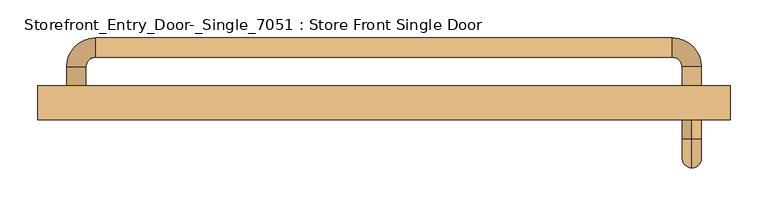
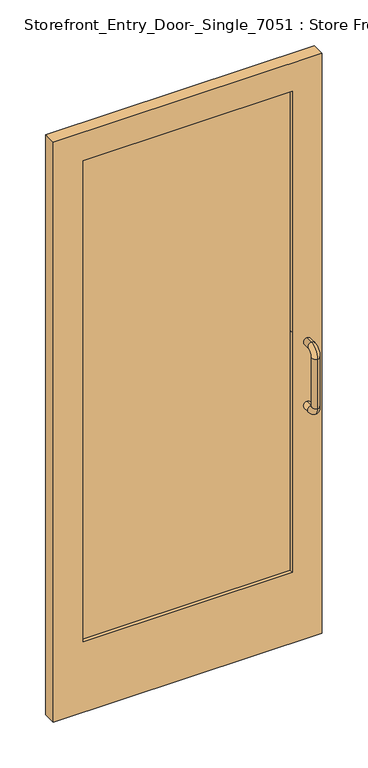
"""IFC4 building model written with IfcOpenShell, lengths in millimetres: door geometry, Storefront_Entry_Door-_Single_7051 : Store Front Single Door."""

from ifc_helpers import new_model, si_unit, point, frame, origin, place, context, project, spatial, polyline, circle_curve, ellipse_curve, trimmed, outline, extrude, source, transform, mapped, element, save
from ifc_brep_helpers import plane_surface, cylinder_surface, revolved_surface, advanced_brep


def storefront_entry_door_single_7051_store_front_single_door_bbd59173(model_context):
    return source(origin(), model_context, "Body", "SolidModel", [
        advanced_brep(
        [(406.4, -50.8, 1054.1), (406.4, -50.8, 1079.5), (406.4, -76.2, 1079.5), (406.4, -76.2, 1054.1), (406.4, -114.3, 1041.4), (406.4, -88.9, 1041.4), (406.4, -114.3, 863.6), (406.4, -88.9, 863.6), (406.4, -76.2, 825.5), (406.4, -76.2, 850.9), (406.4, -50.8, 850.9), (406.4, -50.8, 825.5)],
        [
            (0, 1, circle_curve(frame((406.4, -50.8, 1066.8), z_axis=(0.0, 1.0, 0.0), x_axis=(0.0, 0.0, 1.0)), 12.7)),
            (1, 0, circle_curve(frame((406.4, -50.8, 1066.8), z_axis=(0.0, 1.0, 0.0), x_axis=(0.0, 0.0, 1.0)), 12.7)),
            (1, 2),
            (2, 3, circle_curve(frame((406.4, -76.2, 1066.8), z_axis=(0.0, 1.0, 0.0), x_axis=(0.0, 0.0, 1.0)), 12.7)),
            (3, 0),
            (3, 2, circle_curve(frame((406.4, -76.2, 1066.8), z_axis=(0.0, 1.0, 0.0), x_axis=(0.0, 0.0, 1.0)), 12.7)),
            (4, 5, circle_curve(frame((406.4, -101.6, 1041.4), z_axis=(0.0, 0.0, 1.0), x_axis=(0.0, -1.0, 0.0)), 12.7)),
            (5, 3, circle_curve(frame((406.4, -76.2, 1041.4), z_axis=(-1.0, 0.0, 0.0), x_axis=(0.0, 0.0, 1.0)), 12.7)),
            (2, 4, circle_curve(frame((406.4, -76.2, 1041.4), z_axis=(1.0, 0.0, 0.0), x_axis=(0.0, 0.0, 1.0)), 38.1)),
            (5, 4, circle_curve(frame((406.4, -101.6, 1041.4), z_axis=(0.0, 0.0, 1.0), x_axis=(0.0, -1.0, 0.0)), 12.7)),
            (4, 6),
            (6, 7, circle_curve(frame((406.4, -101.6, 863.6), z_axis=(0.0, 0.0, 1.0), x_axis=(0.0, -1.0, 0.0)), 12.7)),
            (7, 5),
            (7, 6, circle_curve(frame((406.4, -101.6, 863.6), z_axis=(0.0, 0.0, 1.0), x_axis=(0.0, -1.0, 0.0)), 12.7)),
            (8, 9, circle_curve(frame((406.4, -76.2, 838.2), z_axis=(0.0, -1.0, 0.0), x_axis=(0.0, 0.0, -1.0)), 12.7)),
            (9, 7, circle_curve(frame((406.4, -76.2, 863.6), z_axis=(-1.0, 0.0, 0.0), x_axis=(0.0, -1.0, 0.0)), 12.7)),
            (6, 8, circle_curve(frame((406.4, -76.2, 863.6), z_axis=(1.0, 0.0, 0.0), x_axis=(0.0, -1.0, 0.0)), 38.1)),
            (9, 8, circle_curve(frame((406.4, -76.2, 838.2), z_axis=(0.0, -1.0, 0.0), x_axis=(0.0, 0.0, -1.0)), 12.7)),
            (10, 11, circle_curve(frame((406.4, -50.8, 838.2), z_axis=(0.0, 1.0, 0.0), x_axis=(0.0, 0.0, -1.0)), 12.7)),
            (11, 10, circle_curve(frame((406.4, -50.8, 838.2), z_axis=(0.0, 1.0, 0.0), x_axis=(0.0, 0.0, -1.0)), 12.7)),
            (8, 11),
            (10, 9),
        ],
        [
            plane_surface(frame((406.4, -50.8, 1066.8), z_axis=(0.0, 1.0, 0.0), x_axis=(1.0, 0.0, 0.0))),
            cylinder_surface(frame((406.4, -50.8, 1066.8), z_axis=(0.0, 1.0, 0.0), x_axis=(0.0, 0.0, 1.0)), 12.7),
            revolved_surface(trimmed(ellipse_curve(frame((406.4, -76.2, 1066.8), z_axis=(0.0, -1.0, 0.0), x_axis=(0.0, 0.0, 1.0)), 12.7, 12.7), [point((406.4, -76.2, 1054.1))], [point((406.4, -76.2, 1079.5))], True, "CARTESIAN"), (406.4, -76.2, 1041.4), (-1.0, 0.0, 0.0)),
            revolved_surface(trimmed(ellipse_curve(frame((406.4, -76.2, 1066.8), z_axis=(0.0, -1.0, 0.0), x_axis=(0.0, 0.0, 1.0)), 12.7, 12.7), [point((406.4, -76.2, 1079.5))], [point((406.4, -76.2, 1054.1))], True, "CARTESIAN"), (406.4, -76.2, 1041.4), (-1.0, 0.0, 0.0)),
            cylinder_surface(frame((406.4, -101.6, 1041.4), z_axis=(0.0, 0.0, 1.0), x_axis=(0.0, -1.0, 0.0)), 12.7),
            revolved_surface(trimmed(ellipse_curve(frame((406.4, -101.6, 863.6), z_axis=(0.0, 0.0, -1.0), x_axis=(0.0, -1.0, 0.0)), 12.7, 12.7), [point((406.4, -88.9, 863.6))], [point((406.4, -114.3, 863.6))], True, "CARTESIAN"), (406.4, -76.2, 863.6), (-1.0, 0.0, 0.0)),
            revolved_surface(trimmed(ellipse_curve(frame((406.4, -101.6, 863.6), z_axis=(0.0, 0.0, -1.0), x_axis=(0.0, -1.0, 0.0)), 12.7, 12.7), [point((406.4, -114.3, 863.6))], [point((406.4, -88.9, 863.6))], True, "CARTESIAN"), (406.4, -76.2, 863.6), (-1.0, 0.0, 0.0)),
            plane_surface(frame((406.4, -50.8, 838.2), z_axis=(0.0, 1.0, 0.0), x_axis=(1.0, 0.0, 0.0))),
            cylinder_surface(frame((406.4, -76.2, 838.2), z_axis=(0.0, -1.0, 0.0), x_axis=(0.0, 0.0, -1.0)), 12.7),
        ],
        [
            (0, [[1, 2]]),
            (1, [[3, 4, 5, -2]]),
            (1, [[-5, 6, -3, -1]]),
            (2, [[7, 8, -4, 9]]),
            (3, [[10, -9, -6, -8]]),
            (4, [[11, 12, 13, -7]]),
            (4, [[-13, 14, -11, -10]]),
            (5, [[15, 16, -12, 17]]),
            (6, [[18, -17, -14, -16]]),
            (7, [[19, 20]]),
            (8, [[21, -19, 22, -15]]),
            (8, [[-22, -20, -21, -18]]),
        ],
    ),
        advanced_brep(
        [(393.7, -6.35, 1066.8), (419.1, -6.35, 1066.8), (419.1, 19.05, 1066.8), (393.7, 19.05, 1066.8), (381.0, 57.15, 1066.8), (381.0, 31.75, 1066.8), (-381.0, 57.15, 1066.8), (-381.0, 31.75, 1066.8), (-419.1, 19.05, 1066.8), (-393.7, 19.05, 1066.8), (-393.7, -6.35, 1066.8), (-419.1, -6.35, 1066.8)],
        [
            (0, 1, circle_curve(frame((406.4, -6.35, 1066.8), z_axis=(0.0, -1.0, 0.0), x_axis=(1.0, 0.0, 0.0)), 12.7)),
            (1, 0, circle_curve(frame((406.4, -6.35, 1066.8), z_axis=(0.0, -1.0, 0.0), x_axis=(1.0, 0.0, 0.0)), 12.7)),
            (1, 2),
            (2, 3, circle_curve(frame((406.4, 19.05, 1066.8), z_axis=(0.0, -1.0, 0.0), x_axis=(1.0, 0.0, 0.0)), 12.7)),
            (3, 0),
            (3, 2, circle_curve(frame((406.4, 19.05, 1066.8), z_axis=(0.0, -1.0, 0.0), x_axis=(1.0, 0.0, 0.0)), 12.7)),
            (4, 5, circle_curve(frame((381.0, 44.45, 1066.8), z_axis=(1.0, 0.0, 0.0), x_axis=(0.0, 1.0, 0.0)), 12.7)),
            (5, 3, circle_curve(frame((381.0, 19.05, 1066.8), z_axis=(0.0, 0.0, -1.0), x_axis=(1.0, 0.0, 0.0)), 12.7)),
            (2, 4, circle_curve(frame((381.0, 19.05, 1066.8), z_axis=(0.0, 0.0, 1.0), x_axis=(1.0, 0.0, 0.0)), 38.1)),
            (5, 4, circle_curve(frame((381.0, 44.45, 1066.8), z_axis=(1.0, 0.0, 0.0), x_axis=(0.0, 1.0, 0.0)), 12.7)),
            (4, 6),
            (6, 7, circle_curve(frame((-381.0, 44.45, 1066.8), z_axis=(1.0, 0.0, 0.0), x_axis=(0.0, 1.0, 0.0)), 12.7)),
            (7, 5),
            (7, 6, circle_curve(frame((-381.0, 44.45, 1066.8), z_axis=(1.0, 0.0, 0.0), x_axis=(0.0, 1.0, 0.0)), 12.7)),
            (8, 9, circle_curve(frame((-406.4, 19.05, 1066.8), z_axis=(0.0, 1.0, 0.0), x_axis=(-1.0, 0.0, 0.0)), 12.7)),
            (9, 7, circle_curve(frame((-381.0, 19.05, 1066.8), z_axis=(0.0, 0.0, -1.0), x_axis=(0.0, 1.0, 0.0)), 12.7)),
            (6, 8, circle_curve(frame((-381.0, 19.05, 1066.8), z_axis=(0.0, 0.0, 1.0), x_axis=(0.0, 1.0, 0.0)), 38.1)),
            (9, 8, circle_curve(frame((-406.4, 19.05, 1066.8), z_axis=(0.0, 1.0, 0.0), x_axis=(-1.0, 0.0, 0.0)), 12.7)),
            (10, 11, circle_curve(frame((-406.4, -6.35, 1066.8), z_axis=(0.0, -1.0, 0.0), x_axis=(-1.0, 0.0, 0.0)), 12.7)),
            (11, 10, circle_curve(frame((-406.4, -6.35, 1066.8), z_axis=(0.0, -1.0, 0.0), x_axis=(-1.0, 0.0, 0.0)), 12.7)),
            (8, 11),
            (10, 9),
        ],
        [
            plane_surface(frame((406.4, -6.35, 1066.8), z_axis=(0.0, -1.0, 0.0), x_axis=(0.0, 0.0, 1.0))),
            cylinder_surface(frame((406.4, -6.35, 1066.8), z_axis=(0.0, -1.0, 0.0), x_axis=(1.0, 0.0, 0.0)), 12.7),
            revolved_surface(trimmed(ellipse_curve(frame((406.4, 19.05, 1066.8), z_axis=(0.0, 1.0, 0.0), x_axis=(1.0, 0.0, 0.0)), 12.7, 12.7), [point((393.7, 19.05, 1066.8))], [point((419.1, 19.05, 1066.8))], True, "CARTESIAN"), (381.0, 19.05, 1066.8), (0.0, 0.0, -1.0)),
            revolved_surface(trimmed(ellipse_curve(frame((406.4, 19.05, 1066.8), z_axis=(0.0, 1.0, 0.0), x_axis=(1.0, 0.0, 0.0)), 12.7, 12.7), [point((419.1, 19.05, 1066.8))], [point((393.7, 19.05, 1066.8))], True, "CARTESIAN"), (381.0, 19.05, 1066.8), (0.0, 0.0, -1.0)),
            cylinder_surface(frame((381.0, 44.45, 1066.8), z_axis=(1.0, 0.0, 0.0), x_axis=(0.0, 1.0, 0.0)), 12.7),
            revolved_surface(trimmed(ellipse_curve(frame((-381.0, 44.45, 1066.8), z_axis=(-1.0, 0.0, 0.0), x_axis=(0.0, 1.0, 0.0)), 12.7, 12.7), [point((-381.0, 31.75, 1066.8))], [point((-381.0, 57.15, 1066.8))], True, "CARTESIAN"), (-381.0, 19.05, 1066.8), (0.0, 0.0, -1.0)),
            revolved_surface(trimmed(ellipse_curve(frame((-381.0, 44.45, 1066.8), z_axis=(-1.0, 0.0, 0.0), x_axis=(0.0, 1.0, 0.0)), 12.7, 12.7), [point((-381.0, 57.15, 1066.8))], [point((-381.0, 31.75, 1066.8))], True, "CARTESIAN"), (-381.0, 19.05, 1066.8), (0.0, 0.0, -1.0)),
            plane_surface(frame((-406.4, -6.35, 1066.8), z_axis=(0.0, -1.0, 0.0), x_axis=(0.0, 0.0, 1.0))),
            cylinder_surface(frame((-406.4, 19.05, 1066.8), z_axis=(0.0, 1.0, 0.0), x_axis=(-1.0, 0.0, 0.0)), 12.7),
        ],
        [
            (0, [[1, 2]]),
            (1, [[3, 4, 5, -2]]),
            (1, [[-5, 6, -3, -1]]),
            (2, [[7, 8, -4, 9]]),
            (3, [[10, -9, -6, -8]]),
            (4, [[11, 12, 13, -7]]),
            (4, [[-13, 14, -11, -10]]),
            (5, [[15, 16, -12, 17]]),
            (6, [[18, -17, -14, -16]]),
            (7, [[19, 20]]),
            (8, [[21, -19, 22, -15]]),
            (8, [[-22, -20, -21, -18]]),
        ],
    ),
        extrude(outline(polyline([(355.6, -19.05), (355.6, -38.1), (-355.6, -38.1), (-355.6, -19.05), (355.6, -19.05)])), frame((0.0, 0.0, 254.0), z_axis=(0.0, 0.0, 1.0), x_axis=(1.0, 0.0, 0.0)), (0.0, 0.0, 1.0), 1727.2),
        extrude(outline(polyline([(2082.8, 457.2), (2082.8, -457.2), (0.0, -457.2), (0.0, 457.2), (2082.8, 457.2)]), holes=[polyline([(1981.2, -355.6), (1981.2, 355.6), (254.0, 355.6), (254.0, -355.6), (1981.2, -355.6)])]), frame((0.0, -50.8, 0.0), z_axis=(0.0, 1.0, 0.0), x_axis=(0.0, 0.0, 1.0)), (0.0, 0.0, 1.0), 44.45),
    ])


if __name__ == "__main__":
    model = new_model("IFC4")
    model_context = context("Model", 3, world=origin())
    ifc_project = project(units=[si_unit("LENGTHUNIT", "METRE", prefix="MILLI")], contexts=[model_context])
    site = spatial("IfcSite", under=ifc_project)
    building = spatial("IfcBuilding", under=site)
    placement = place(None, origin())
    storefront_entry_door_single_7051_store_front_single_door_shape = storefront_entry_door_single_7051_store_front_single_door_bbd59173(model_context)
    element("IfcDoor", 1, ObjectType="Storefront_Entry_Door-_Single_7051 : Store Front Single Door", at=placement, inside=building, context=model_context, shape_type="MappedRepresentation", body=[
        mapped(storefront_entry_door_single_7051_store_front_single_door_shape, transform((0.0, 0.0, 0.0), x_axis=(1.0, 0.0, 0.0), y_axis=(0.0, 1.0, 0.0), z_axis=(0.0, 0.0, 1.0))),
    ])
    save(model, "model.ifc")

# Revit data of these elements
# Type "Storefront_Entry_Door-_Single_7051 : Store Front Single Door"
#   Type Mark = "20"
#   Assembly Code = "B2030110"
#   Top Rail = 0' - 4"
#   Side Rail = 0' - 4"
#   Rail Height AFF = 3' - 6"
#   Offset = 0' - 2"
#   Bottom Rail Width = 0' - 10"
#   Material = storefront color
#   Glazing Material = Glass
#   Function = (empty or 0)
# Element 1 (IfcDoor, "Storefront_Entry_Door-_Single_7051 : Store Front Single Door")
#   Materials on its faces: "storefront color", "Glass"
# Materials
#   "storefront color": class "Generic", colour RGB 26 26 30, transparency 0, Cost = 0
#   "Glass": class "Glass", colour RGB 218 227 224, transparency 0.85, Description = "Soda Lime Glass", Cost = 0
